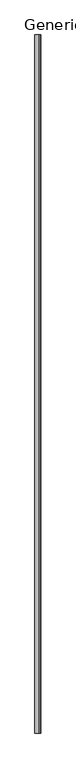
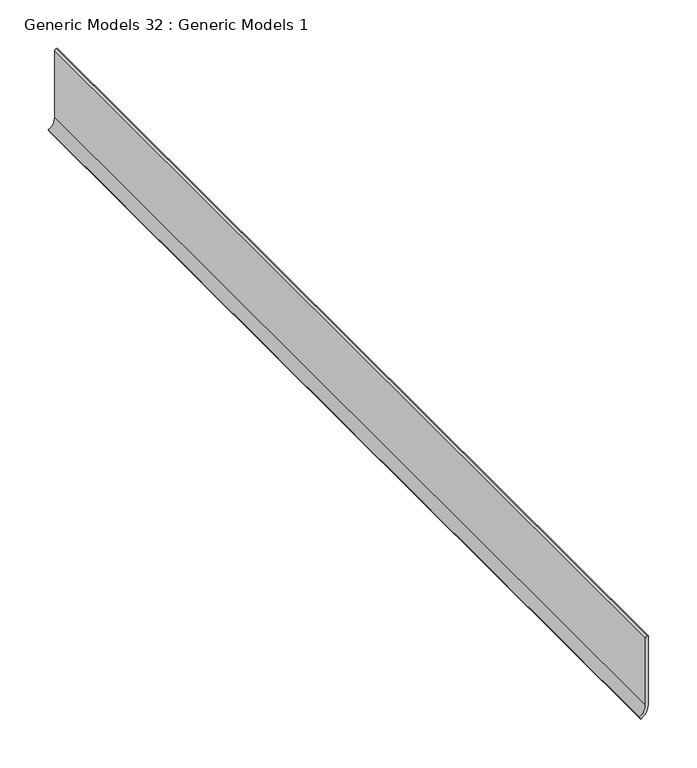
"""IFC4 building model written with IfcOpenShell, lengths in millimetres: proxy geometry, Generic Models 32 : Generic Models 1."""

from ifc_helpers import new_model, si_unit, point, frame, frame_2d, origin, place, context, project, spatial, polyline, circle_curve, trimmed, segment, composite_curve, outline, extrude, source, transform, mapped, element, save


def generic_models_32_generic_models_1_fdd6cadd(model_context):
    return source(origin(), model_context, "Body", "SweptSolid", [
        extrude(outline(composite_curve([segment(polyline([(73.749588, 48367.3939813), (73.749588, 48366.3057831)]), True, "CONTINUOUS"), segment(trimmed(circle_curve(frame_2d((71.6627862, 48366.3057831)), 2.0868018), [point((73.749588, 48366.3057831))], [point((71.6627862, 48364.2189813))], False, "CARTESIAN"), True, "CONTINUOUS"), segment(polyline([(71.6627862, 48364.2189813), (-12.4007813, 48364.2189813)]), True, "CONTINUOUS"), segment(trimmed(circle_curve(frame_2d((-12.4007813, 48349.5542845)), 14.6646968), [point((-12.4007813, 48364.2189813))], [point((-25.1007813, 48356.8866329))], True, "CARTESIAN"), True, "CONTINUOUS"), segment(polyline([(-25.1007813, 48356.8866329), (-27.850412, 48358.4741329)]), True, "CONTINUOUS"), segment(trimmed(circle_curve(frame_2d((-12.4007813, 48349.5542845)), 17.8396968), [point((-27.850412, 48358.4741329))], [point((-12.4007813, 48367.3939813))], False, "CARTESIAN"), True, "CONTINUOUS"), segment(polyline([(-12.4007813, 48367.3939813), (73.749588, 48367.3939813)]), True, "CONTINUOUS")], self_intersect=False)), frame((0.0, 0.0, 0.0), z_axis=(0.0, 1.0, 0.0), x_axis=(0.0, 0.0, 1.0)), (0.0, 0.0, 1.0), 1219.2),
    ])


if __name__ == "__main__":
    model = new_model("IFC4")
    model_context = context("Model", 3, world=origin())
    ifc_project = project(units=[si_unit("LENGTHUNIT", "METRE", prefix="MILLI")], contexts=[model_context])
    site = spatial("IfcSite", under=ifc_project)
    building = spatial("IfcBuilding", under=site)
    placement = place(None, origin())
    generic_models_32_generic_models_1_shape = generic_models_32_generic_models_1_fdd6cadd(model_context)
    element("IfcBuildingElementProxy", 1, Name="Generic Models 32 : Generic Models 1", ObjectType="Generic Models 32 : Generic Models 1", at=placement, inside=building, context=model_context, shape_type="MappedRepresentation", body=[
        mapped(generic_models_32_generic_models_1_shape, transform((0.0, 0.0, 0.0), x_axis=(1.0, 0.0, 0.0), y_axis=(0.0, 1.0, 0.0), z_axis=(0.0, 0.0, 1.0))),
    ])
    save(model, "model.ifc")

# Revit data of these elements
# Element 1 (IfcBuildingElementProxy, "Generic Models 32 : Generic Models 1")
#   Materials on its faces: "BASE AS SCHEDULED"
# Materials
#   "BASE AS SCHEDULED": class "Generic", colour RGB 120 120 120, transparency 0, Cost = 0
